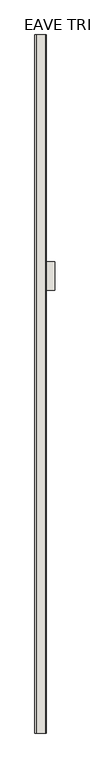
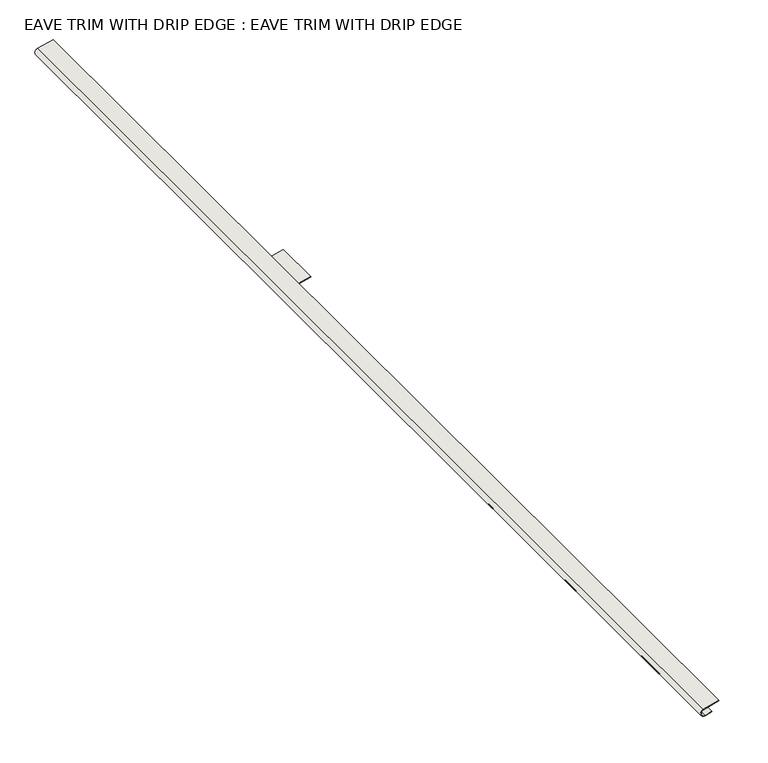
"""IFC4 building model written with IfcOpenShell, lengths in millimetres: wall geometry, EAVE TRIM WITH DRIP EDGE : EAVE TRIM WITH DRIP EDGE."""

from ifc_helpers import new_model, si_unit, point, frame, frame_2d, origin, place, context, project, spatial, polyline, circle_curve, trimmed, segment, composite_curve, outline, extrude, source, transform, mapped, element, save


def eave_trim_with_drip_edge_eave_trim_with_drip_edge_45c72aa3(model_context):
    return source(origin(), model_context, "Body", "SweptSolid", [
        extrude(outline(composite_curve([segment(polyline([(2364.6781787, 17370.0689283), (2392.9342544, 17363.0238974), (2386.7736072, 17338.3813086)]), True, "CONTINUOUS"), segment(trimmed(circle_curve(frame_2d((2387.5436578, 17338.1887959)), 0.79375), [point((2386.7736072, 17338.3813086))], [point((2388.3137084, 17337.9962833))], True, "CARTESIAN"), True, "CONTINUOUS"), segment(polyline([(2388.3137084, 17337.9962833), (2409.8789073, 17424.2570789), (2411.4190085, 17423.8720536), (2389.8538096, 17337.611258)]), True, "CONTINUOUS"), segment(trimmed(circle_curve(frame_2d((2387.5436578, 17338.1887959)), 2.38125), [point((2389.8538096, 17337.611258))], [point((2385.2335059, 17338.7663339))], False, "CARTESIAN"), True, "CONTINUOUS"), segment(polyline([(2385.2335059, 17338.7663339), (2391.0088842, 17361.8678469), (2364.8395923, 17368.3925842), (2347.574429, 17360.3417063)]), True, "CONTINUOUS"), segment(trimmed(circle_curve(frame_2d((2346.5680692, 17362.4998517)), 2.38125), [point((2347.574429, 17360.3417063))], [point((2345.5617095, 17364.6579972))], False, "CARTESIAN"), True, "CONTINUOUS"), segment(polyline([(2345.5617095, 17364.6579972), (2350.0325947, 17366.7428052), (2350.7035012, 17365.3040415), (2346.232616, 17363.2192335)]), True, "CONTINUOUS"), segment(trimmed(circle_curve(frame_2d((2346.5680692, 17362.4998517)), 0.79375), [point((2346.232616, 17363.2192335))], [point((2346.9035225, 17361.7804699))], True, "CARTESIAN"), True, "CONTINUOUS"), segment(polyline([(2346.9035225, 17361.7804699), (2364.6781787, 17370.0689283)]), True, "CONTINUOUS")], self_intersect=False)), frame((0.0, -1256.0384634, 0.0), z_axis=(0.0, 1.0, 0.0), x_axis=(0.0, 0.0, 1.0)), (0.0, 0.0, 1.0), 139.7),
        extrude(outline(composite_curve([segment(polyline([(2398.5017334, 17337.0845893), (2409.8897838, 17382.6367909), (2411.429885, 17382.2517656), (2400.0418346, 17336.699564)]), True, "CONTINUOUS"), segment(trimmed(circle_curve(frame_2d((2389.2611261, 17339.3947411)), 11.1125), [point((2400.0418346, 17336.699564))], [point((2378.4804175, 17342.0899183))], False, "CARTESIAN"), True, "CONTINUOUS"), segment(polyline([(2378.4804175, 17342.0899183), (2383.4504448, 17361.9700271), (2384.990546, 17361.5850018), (2380.0205188, 17341.704893)]), True, "CONTINUOUS"), segment(trimmed(circle_curve(frame_2d((2389.2611261, 17339.3947411)), 9.525), [point((2380.0205188, 17341.704893))], [point((2398.5017334, 17337.0845893))], True, "CARTESIAN"), True, "CONTINUOUS")], self_intersect=False)), frame((0.0, -3415.0384634, 0.0), z_axis=(0.0, 1.0, 0.0), x_axis=(0.0, 0.0, 1.0)), (0.0, 0.0, 1.0), 3403.6),
    ])


if __name__ == "__main__":
    model = new_model("IFC4")
    model_context = context("Model", 3, world=origin())
    ifc_project = project(units=[si_unit("LENGTHUNIT", "METRE", prefix="MILLI")], contexts=[model_context])
    site = spatial("IfcSite", under=ifc_project)
    building = spatial("IfcBuilding", under=site)
    placement = place(None, origin())
    eave_trim_with_drip_edge_eave_trim_with_drip_edge_shape = eave_trim_with_drip_edge_eave_trim_with_drip_edge_45c72aa3(model_context)
    element("IfcWall", 1, ObjectType="EAVE TRIM WITH DRIP EDGE : EAVE TRIM WITH DRIP EDGE", at=placement, inside=building, context=model_context, shape_type="MappedRepresentation", body=[
        mapped(eave_trim_with_drip_edge_eave_trim_with_drip_edge_shape, transform((0.0, 0.0, 0.0), x_axis=(1.0, 0.0, 0.0), y_axis=(0.0, 1.0, 0.0), z_axis=(0.0, 0.0, 1.0))),
    ])
    save(model, "model.ifc")

# Revit data of these elements
# Element 1 (IfcWall, "EAVE TRIM WITH DRIP EDGE : EAVE TRIM WITH DRIP EDGE")
#   Materials on its faces: "EAVE TRIM W/ DRIP EDGE", "STANDING SEAM METAL ROOF (SPEC. TBD)"
# Materials
#   "EAVE TRIM W/ DRIP EDGE": class "Generic", colour RGB 195 195 195, transparency 0, Cost = 0
#   "STANDING SEAM METAL ROOF (SPEC. TBD)": class "Paint", colour RGB 104 104 104, transparency 0, Cost = 0
